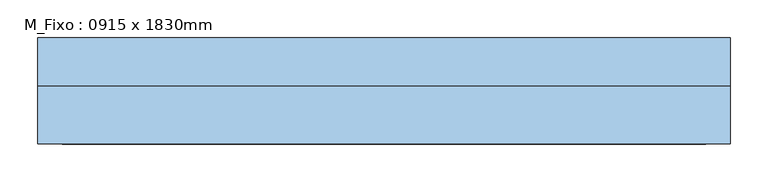
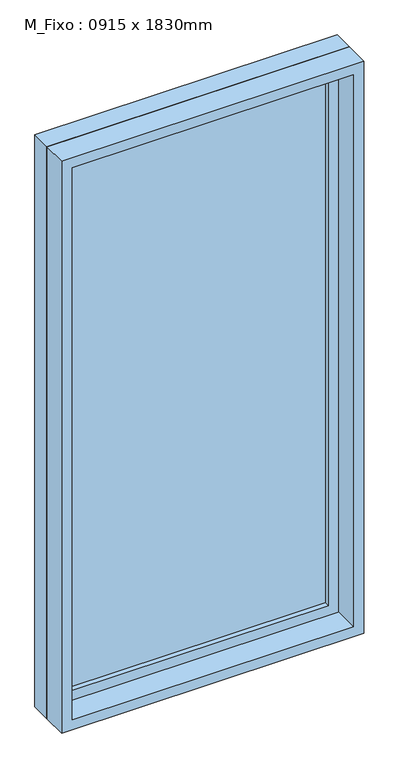
"""IFC4 building model written with IfcOpenShell, lengths in millimetres: window geometry, M_Fixo : 0915 x 1830mm."""

from ifc_helpers import new_model, si_unit, frame, origin, place, context, project, spatial, polyline, outline, extrude, source, transform, mapped, element, save


def m_fixo_0915_x_1830mm_1cb826ad(model_context):
    return source(origin(), model_context, "Body", "SweptSolid", [
        extrude(outline(polyline([(-394.5, 48.0), (394.5, 48.0), (394.5, 36.0), (-394.5, 36.0), (-394.5, 48.0)])), frame((0.0, 0.0, 368.0), z_axis=(0.0, 0.0, 1.0), x_axis=(1.0, 0.0, 0.0)), (0.0, 0.0, 1.0), 1704.0),
        extrude(outline(polyline([(2116.0, -438.5), (324.0, -438.5), (324.0, 438.5), (2116.0, 438.5), (2116.0, -438.5)]), holes=[polyline([(2072.0, -394.5), (2072.0, 394.5), (368.0, 394.5), (368.0, -394.5), (2072.0, -394.5)])]), frame((0.0, 20.0, 0.0), z_axis=(0.0, 1.0, 0.0), x_axis=(0.0, 0.0, 1.0)), (0.0, 0.0, 1.0), 44.0),
        extrude(outline(polyline([(2135.0, -457.5), (305.0, -457.5), (305.0, 457.5), (2135.0, 457.5), (2135.0, -457.5)]), holes=[polyline([(2116.0, -438.5), (2116.0, 438.5), (324.0, 438.5), (324.0, -438.5), (2116.0, -438.5)])]), frame((0.0, 20.0, 0.0), z_axis=(0.0, 1.0, 0.0), x_axis=(0.0, 0.0, 1.0)), (0.0, 0.0, 1.0), 63.0),
        extrude(outline(polyline([(2135.0, -457.5), (305.0, -457.5), (305.0, 457.5), (2135.0, 457.5), (2135.0, -457.5)]), holes=[polyline([(2103.0, -425.5), (2103.0, 425.5), (337.0, 425.5), (337.0, -425.5), (2103.0, -425.5)])]), frame((0.0, -57.0, 0.0), z_axis=(0.0, 1.0, 0.0), x_axis=(0.0, 0.0, 1.0)), (0.0, 0.0, 1.0), 77.0),
    ])


if __name__ == "__main__":
    model = new_model("IFC4")
    model_context = context("Model", 3, world=origin())
    ifc_project = project(units=[si_unit("LENGTHUNIT", "METRE", prefix="MILLI")], contexts=[model_context])
    site = spatial("IfcSite", under=ifc_project)
    building = spatial("IfcBuilding", under=site)
    placement = place(None, origin())
    m_fixo_0915_x_1830mm_shape = m_fixo_0915_x_1830mm_1cb826ad(model_context)
    element("IfcWindow", 1, ObjectType="M_Fixo : 0915 x 1830mm", at=placement, inside=building, context=model_context, shape_type="MappedRepresentation", body=[
        mapped(m_fixo_0915_x_1830mm_shape, transform((0.0, 0.0, 0.0), x_axis=(1.0, 0.0, 0.0), y_axis=(0.0, 1.0, 0.0), z_axis=(0.0, 0.0, 1.0))),
    ])
    save(model, "model.ifc")

# Revit data of these elements
# Type "M_Fixo : 0915 x 1830mm"
#   Type Mark = "18"
#   Construction Type Id = "GSP4R"
#   Analytic Construction = "Vidraça única Pilkington 1/8 pol"
#   Visual Light Transmittance = 0.9
#   Thermal Resistance (R) = 0.271106 (m²·K)/W
#   Solar Heat Gain Coefficient = 0.78
#   Heat Transfer Coefficient (U) = 3.6886 W/(m²·K)
#   Height = 1.83 m
#   Altura-padrão do peitoril = 0.305 m
#   Width = 0.915 m
#   Janela aplicada = 0.019 m
#   Define Thermal Properties by = 1
#   Define Thermal Properties by = 1
#   Material da estrutura externa = Caixilho
#   Material da estrutura interna = Caixilho
#   Material do painel de vidro = Vidro
#   Caixilho = Caixilho
#   Wall Closure = (empty or 0)
# Element 1 (IfcWindow, "M_Fixo : 0915 x 1830mm")
#   Materials on its faces: "Caixilho", "Vidro"
# Materials
#   "Caixilho": class "Madeira", colour RGB 224 178 126, transparency 0, Cost = 0
#   "Vidro": class "Vidro", colour RGB 0 128 192, transparency 0.9, Description = "Vidro de sílica", Cost = 0
